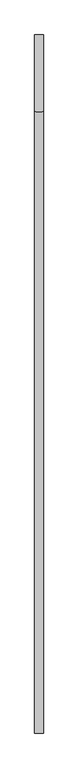
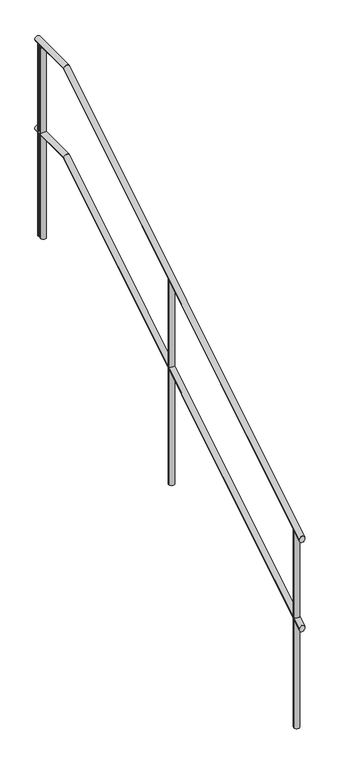
"""IFC4 building model written with IfcOpenShell, lengths in millimetres: railing geometry."""

import ifcopenshell
import ifcopenshell.guid

model = None  # the IFC model being written
_history = None  # IfcOwnerHistory: only IFC2X3 demands one
_inside = {}  # id of a spatial element -> (the spatial element, [elements in it])
_under = {}  # id of a project, library or spatial element -> (it, [spatial elements below it])
_declared = {}  # id of a project -> (the project, [libraries it declares])
_typed = {}  # id of a type object -> (the type object, [elements of that type])
_made_of = {}  # id of a material, layer set ... -> (it, [elements and type objects made of it])


def new_model(schema):
    """Start an empty IFC model of exactly this schema.

    Asked for "IFC4X3", IfcOpenShell would pick the latest addendum, in which some entities
    have other attributes; the version numbers below select the first issue.
    IFC2X3 requires an IfcOwnerHistory on every rooted entity: one is made here for all.
    """
    global model, _history
    if schema == "IFC4X3":
        model = ifcopenshell.file(schema_version=(4, 3, 0, 0))
    else:
        model = ifcopenshell.file(schema=schema)
    _inside.clear()
    _under.clear()
    _declared.clear()
    _typed.clear()
    _made_of.clear()
    _history = None
    if model.schema == "IFC2X3":
        org = make("IfcOrganization", Name="unknown")
        user = make(
            "IfcPersonAndOrganization",
            ThePerson=make("IfcPerson", FamilyName="unknown"),
            TheOrganization=org,
        )
        app = make(
            "IfcApplication",
            ApplicationDeveloper=org,
            Version="unknown",
            ApplicationFullName="unknown",
            ApplicationIdentifier="unknown",
        )
        _history = make(
            "IfcOwnerHistory",
            OwningUser=user,
            OwningApplication=app,
            ChangeAction="ADDED",
            CreationDate=0,
        )
    return model


def make(cls, **values):
    """One entity of the class cls with the attributes given. An attribute that is None is left unset."""
    return model.create_entity(
        cls, **{name: value for name, value in values.items() if value is not None}
    )


def rooted(cls, **values):
    """An entity with a GlobalId (a new one), such as an element, a storey or a relation."""
    return make(cls, GlobalId=ifcopenshell.guid.new(), OwnerHistory=_history, **values)


def si_unit(unit_type, name, prefix=None):
    """IfcSIUnit, for example si_unit("LENGTHUNIT", "METRE", prefix="MILLI")."""
    return make("IfcSIUnit", UnitType=unit_type, Prefix=prefix, Name=name)


def assignment(units):
    """IfcUnitAssignment: the units of a project."""
    return None if units is None else make("IfcUnitAssignment", Units=units)


def point(xyz):
    """IfcCartesianPoint."""
    return None if xyz is None else make("IfcCartesianPoint", Coordinates=xyz)


def direction(xyz):
    """IfcDirection."""
    return None if xyz is None else make("IfcDirection", DirectionRatios=xyz)


def frame(location, z_axis=None, x_axis=None):
    """IfcAxis2Placement3D, a coordinate frame: its origin and axes. An axis left out is left unset."""
    return make(
        "IfcAxis2Placement3D",
        Location=point(location),
        Axis=direction(z_axis),
        RefDirection=direction(x_axis),
    )


def frame_2d(location, x_axis=None):
    """IfcAxis2Placement2D, a coordinate frame in the plane: its origin and x axis."""
    return make(
        "IfcAxis2Placement2D", Location=point(location), RefDirection=direction(x_axis)
    )


def origin():
    """The frame at (0, 0, 0) with its axes left unset."""
    return frame((0.0, 0.0, 0.0))


def place(relative_to, where):
    """IfcLocalPlacement: puts the frame where relative to a parent placement (None: the world)."""
    return make(
        "IfcLocalPlacement", PlacementRelTo=relative_to, RelativePlacement=where
    )


def context(
    kind, dimensions, precision=None, world=None, true_north=None, identifier=None
):
    """IfcGeometricRepresentationContext, for example the 3D "Model" context."""
    return make(
        "IfcGeometricRepresentationContext",
        ContextIdentifier=identifier,
        ContextType=kind,
        CoordinateSpaceDimension=dimensions,
        Precision=precision,
        WorldCoordinateSystem=world,
        TrueNorth=true_north,
    )


def project(units=None, contexts=None):
    """IfcProject with its units and contexts."""
    return rooted(
        "IfcProject",
        Name="project",
        RepresentationContexts=contexts,
        UnitsInContext=assignment(units),
    )


def spatial(cls, under=None, at=None, **own):
    """A site, building, storey or space (cls), placed at a placement, below another one or the project."""
    s = rooted(cls, ObjectPlacement=at, **own)
    if under is not None:
        _under.setdefault(under.id(), (under, []))[1].append(s)
    return s


def circle_curve(where, radius):
    """IfcCircle in the frame where."""
    return make("IfcCircle", Position=where, Radius=radius)


def ellipse_curve(where, semi_axis1, semi_axis2):
    """IfcEllipse in the frame where."""
    return make(
        "IfcEllipse", Position=where, SemiAxis1=semi_axis1, SemiAxis2=semi_axis2
    )


def trimmed(basis, trim1, trim2, sense, master):
    """IfcTrimmedCurve: the piece of a basis curve between two trims."""
    return make(
        "IfcTrimmedCurve",
        BasisCurve=basis,
        Trim1=trim1,
        Trim2=trim2,
        SenseAgreement=sense,
        MasterRepresentation=master,
    )


def segment(curve, same_sense, transition):
    """IfcCompositeCurveSegment."""
    return make(
        "IfcCompositeCurveSegment",
        Transition=transition,
        SameSense=same_sense,
        ParentCurve=curve,
    )


def composite_curve(segments, self_intersect=None):
    """IfcCompositeCurve: segments joined end to end."""
    return make("IfcCompositeCurve", Segments=segments, SelfIntersect=self_intersect)


def outline(outer, holes=None, kind="AREA"):
    """IfcArbitraryClosedProfileDef: a profile drawn as a closed curve; with holes, ...WithVoids."""
    if holes is None:
        return make("IfcArbitraryClosedProfileDef", ProfileType=kind, OuterCurve=outer)
    return make(
        "IfcArbitraryProfileDefWithVoids",
        ProfileType=kind,
        OuterCurve=outer,
        InnerCurves=holes,
    )


def extrude(swept, where, along, depth):
    """IfcExtrudedAreaSolid: the profile swept, set in the frame where, extruded along a direction by depth."""
    return make(
        "IfcExtrudedAreaSolid",
        SweptArea=swept,
        Position=where,
        ExtrudedDirection=direction(along),
        Depth=depth,
    )


def shape(context_of_items, identifier, shape_type, items):
    """IfcShapeRepresentation: the items that make up one representation, for example the "Body"."""
    return make(
        "IfcShapeRepresentation",
        ContextOfItems=context_of_items,
        RepresentationIdentifier=identifier,
        RepresentationType=shape_type,
        Items=items,
    )


def source(mapping_origin, context_of_items, identifier, shape_type, items):
    """IfcRepresentationMap: a shape defined once, which mapped items show again and again."""
    return make(
        "IfcRepresentationMap",
        MappingOrigin=mapping_origin,
        MappedRepresentation=shape(context_of_items, identifier, shape_type, items),
    )


def transform(
    local_origin,
    x_axis=None,
    y_axis=None,
    z_axis=None,
    scale=None,
    scale2=None,
    scale3=None,
    uniform=True,
):
    """IfcCartesianTransformationOperator3D, or its non-uniform kind. x_axis, y_axis, z_axis: its Axis1, 2, 3."""
    if uniform:
        return make(
            "IfcCartesianTransformationOperator3D",
            Axis1=direction(x_axis),
            Axis2=direction(y_axis),
            LocalOrigin=point(local_origin),
            Scale=scale,
            Axis3=direction(z_axis),
        )
    return make(
        "IfcCartesianTransformationOperator3DnonUniform",
        Axis1=direction(x_axis),
        Axis2=direction(y_axis),
        LocalOrigin=point(local_origin),
        Scale=scale,
        Axis3=direction(z_axis),
        Scale2=scale2,
        Scale3=scale3,
    )


def mapped(mapping_source, mapping_target):
    """IfcMappedItem: shows the shape of a source again, moved by a transform."""
    return make(
        "IfcMappedItem", MappingSource=mapping_source, MappingTarget=mapping_target
    )


def made_of(thing, what):
    """Note that an element or type object is made of a material, layer set ...; save() writes the relation."""
    if what is not None:
        _made_of.setdefault(what.id(), (what, []))[1].append(thing)
    return thing


def element(
    cls,
    number,
    at=None,
    inside=None,
    cuts=None,
    type_object=None,
    material=None,
    context=None,
    identifier="Body",
    shape_type=None,
    held_by="IfcProductDefinitionShape",
    body=None,
    shapes=None,
    **own,
):
    """One element of the class cls, such as IfcWall. Its Tag is "e" and its number.

    at: its placement. inside: the storey or other place that contains it. cuts: it is an
    opening in that element (IfcRelVoidsElement). A single representation is given by context,
    identifier, shape_type and body (its items); several are given by shapes. held_by: the class
    of the entity that holds the representations. save() writes the other relations.
    """
    e = rooted(cls, Tag="e%d" % number, ObjectPlacement=at, **own)
    if body is not None:
        shapes = [shape(context, identifier, shape_type, body)]
    if shapes is not None:
        e.Representation = make(held_by, Representations=shapes)
    if inside is not None:
        _inside.setdefault(inside.id(), (inside, []))[1].append(e)
    if cuts is not None:
        rooted(
            "IfcRelVoidsElement", RelatingBuildingElement=cuts, RelatedOpeningElement=e
        )
    if type_object is not None:
        _typed.setdefault(type_object.id(), (type_object, []))[1].append(e)
    return made_of(e, material)


def aggregate(whole, parts):
    """IfcRelAggregates: a whole, such as a stair, and the parts it consists of."""
    return rooted("IfcRelAggregates", RelatingObject=whole, RelatedObjects=parts)


def save(model, path):
    """Write the relations noted so far, then the file.

    IfcRelAggregates (storeys below a building ...), IfcRelContainedInSpatialStructure (elements
    in a storey), IfcRelDefinesByType, IfcRelAssociatesMaterial and IfcRelDeclares: one each for
    every whole, place, type object, material and project.
    """
    for whole, parts in _under.values():
        aggregate(whole, parts)
    for where, things in _inside.values():
        rooted(
            "IfcRelContainedInSpatialStructure",
            RelatedElements=things,
            RelatingStructure=where,
        )
    for kind, things in _typed.values():
        rooted("IfcRelDefinesByType", RelatedObjects=things, RelatingType=kind)
    for what, things in _made_of.values():
        rooted("IfcRelAssociatesMaterial", RelatedObjects=things, RelatingMaterial=what)
    for by, libraries in _declared.values():
        rooted("IfcRelDeclares", RelatingContext=by, RelatedDefinitions=libraries)
    model.write(path)


def plane_surface(at):
    """IfcPlane: the flat surface through the origin of the frame at, square to its z axis."""
    return make("IfcPlane", Position=at)


def cylinder_surface(at, radius):
    """IfcCylindricalSurface: all points at the distance radius from the z axis of the frame at."""
    return make("IfcCylindricalSurface", Position=at, Radius=radius)


def advanced_brep(points, edges, surfaces, faces):
    """IfcAdvancedBrep: a solid bounded by faces that lie on surfaces and meet in shared edges.

    An edge is (start, end): straight between two places in points (the first is 0);
    or (start, end, curve); or (start, end, curve, False) where it runs against its curve.
    A face is (place in surfaces, loops), or (place, loops, False) where it looks against
    its surface's normal. A loop lists edges by number (the first is 1), with a minus sign
    where the edge is run from its end to its start. The first loop is the outer one.
    """
    corners = [point(p) for p in points]
    vertices = [make("IfcVertexPoint", VertexGeometry=c) for c in corners]
    made = []
    for start, end, *more in edges:
        made.append(
            make(
                "IfcEdgeCurve",
                EdgeStart=vertices[start],
                EdgeEnd=vertices[end],
                EdgeGeometry=more[0] if more else make("IfcPolyline", Points=[corners[start], corners[end]]),
                SameSense=more[1] if len(more) > 1 else True,
            )
        )
    hull = []
    for where, loops, *sense in faces:
        bounds = []
        for j, loop in enumerate(loops):
            ring = [make("IfcOrientedEdge", EdgeElement=made[abs(k) - 1], Orientation=k > 0) for k in loop]
            bounds.append(
                make(
                    "IfcFaceOuterBound" if j == 0 else "IfcFaceBound",
                    Bound=make("IfcEdgeLoop", EdgeList=ring),
                    Orientation=True,
                )
            )
        hull.append(make("IfcAdvancedFace", Bounds=bounds, FaceSurface=surfaces[where], SameSense=sense[0] if sense else True))
    return make("IfcAdvancedBrep", Outer=make("IfcClosedShell", CfsFaces=hull))


def railing_2704ba66(model_context):
    return source(origin(), model_context, "Body", "SolidModel", [
        advanced_brep(
        [(-1026.0, 45684.2482382, -450.9609787), (-1056.0, 45684.2482382, -450.9609787), (-1026.0, 47848.5050237, 885.0), (-1056.0, 47848.5050237, 885.0), (-1026.0, 48114.2482382, 885.0), (-1056.0, 48114.2482382, 885.0)],
        [
            (0, 1, ellipse_curve(frame((-1041.0, 45684.2482382, -450.9609787), z_axis=(0.0, -1.0, 0.0), x_axis=(0.0, 0.0, -1.0)), 17.6276454, 15.0)),
            (1, 0, ellipse_curve(frame((-1041.0, 45684.2482382, -450.9609787), z_axis=(0.0, -1.0, 0.0), x_axis=(0.0, 0.0, -1.0)), 17.6276454, 15.0)),
            (0, 2),
            (2, 3, ellipse_curve(frame((-1041.0, 47848.5050237, 885.0), z_axis=(0.0, -0.9620125025549409, -0.27300539358770887), x_axis=(0.0, 0.27300539358770864, -0.962012502554941)), 15.5923129, 15.0)),
            (3, 1),
            (3, 2, ellipse_curve(frame((-1041.0, 47848.5050237, 885.0), z_axis=(0.0, -0.9620125025549409, -0.27300539358770887), x_axis=(0.0, 0.27300539358770864, -0.962012502554941)), 15.5923129, 15.0)),
            (4, 5, circle_curve(frame((-1041.0, 48114.2482382, 885.0), z_axis=(0.0, 1.0, 0.0), x_axis=(-1.0, 0.0, 0.0)), 15.0)),
            (5, 4, circle_curve(frame((-1041.0, 48114.2482382, 885.0), z_axis=(0.0, 1.0, 0.0), x_axis=(-1.0, 0.0, 0.0)), 15.0)),
            (2, 4),
            (5, 3),
        ],
        [
            plane_surface(frame((-1041.0, 45684.2482382, -433.3333333), z_axis=(0.0, -1.0, 0.0), x_axis=(0.0, 0.0, 1.0))),
            cylinder_surface(frame((-1041.0, 45692.1272762, -446.097375), z_axis=(0.0, -0.8509361101440404, -0.5252692037926169), x_axis=(-1.0, 0.0, 0.0)), 15.0),
            plane_surface(frame((-1041.0, 48114.2482382, 900.0), z_axis=(0.0, 1.0, 0.0), x_axis=(0.0, 0.0, 1.0))),
            cylinder_surface(frame((-1041.0, 47844.2482382, 885.0), z_axis=(0.0, -1.0, 0.0), x_axis=(-1.0, 0.0, 0.0)), 15.0),
        ],
        [
            (0, [[1, 2]]),
            (1, [[-1, 3, 4, 5]]),
            (1, [[-2, -5, 6, -3]]),
            (2, [[7, 8]]),
            (3, [[-4, 9, -8, 10]]),
            (3, [[-6, -10, -7, -9]]),
        ],
    ),
        advanced_brep(
        [(-1026.0, 45684.2482382, 49.0390213), (-1056.0, 45684.2482382, 49.0390213), (-1026.0, 47848.5050237, 1385.0), (-1056.0, 47848.5050237, 1385.0), (-1026.0, 48114.2482382, 1385.0), (-1056.0, 48114.2482382, 1385.0)],
        [
            (0, 1, ellipse_curve(frame((-1041.0, 45684.2482382, 49.0390213), z_axis=(0.0, -1.0, 0.0), x_axis=(0.0, 0.0, -1.0)), 17.6276454, 15.0)),
            (1, 0, ellipse_curve(frame((-1041.0, 45684.2482382, 49.0390213), z_axis=(0.0, -1.0, 0.0), x_axis=(0.0, 0.0, -1.0)), 17.6276454, 15.0)),
            (0, 2),
            (2, 3, ellipse_curve(frame((-1041.0, 47848.5050237, 1385.0), z_axis=(0.0, -0.9620125025549409, -0.27300539358770887), x_axis=(0.0, 0.27300539358770864, -0.962012502554941)), 15.5923129, 15.0)),
            (3, 1),
            (3, 2, ellipse_curve(frame((-1041.0, 47848.5050237, 1385.0), z_axis=(0.0, -0.9620125025549409, -0.27300539358770887), x_axis=(0.0, 0.27300539358770864, -0.962012502554941)), 15.5923129, 15.0)),
            (4, 5, circle_curve(frame((-1041.0, 48114.2482382, 1385.0), z_axis=(0.0, 1.0, 0.0), x_axis=(-1.0, 0.0, 0.0)), 15.0)),
            (5, 4, circle_curve(frame((-1041.0, 48114.2482382, 1385.0), z_axis=(0.0, 1.0, 0.0), x_axis=(-1.0, 0.0, 0.0)), 15.0)),
            (2, 4),
            (5, 3),
        ],
        [
            plane_surface(frame((-1041.0, 45684.2482382, 66.6666667), z_axis=(0.0, -1.0, 0.0), x_axis=(0.0, 0.0, 1.0))),
            cylinder_surface(frame((-1041.0, 45692.1272762, 53.902625), z_axis=(0.0, -0.8509361101440404, -0.5252692037926169), x_axis=(-1.0, 0.0, 0.0)), 15.0),
            plane_surface(frame((-1041.0, 48114.2482382, 1400.0), z_axis=(0.0, 1.0, 0.0), x_axis=(0.0, 0.0, 1.0))),
            cylinder_surface(frame((-1041.0, 47844.2482382, 1385.0), z_axis=(0.0, -1.0, 0.0), x_axis=(-1.0, 0.0, 0.0)), 15.0),
        ],
        [
            (0, [[1, 2]]),
            (1, [[-1, 3, 4, 5]]),
            (1, [[-2, -5, 6, -3]]),
            (2, [[7, 8]]),
            (3, [[-4, 9, -8, 10]]),
            (3, [[-6, -10, -7, -9]]),
        ],
    ),
        extrude(outline(composite_curve([segment(trimmed(circle_curve(frame_2d((-1041.0, 48084.2482382)), 15.0), [point((-1026.0, 48084.2482382))], [point((-1056.0, 48084.2482382))], False, "CARTESIAN"), True, "CONTINUOUS"), segment(trimmed(circle_curve(frame_2d((-1041.0, 48084.2482382)), 15.0), [point((-1056.0, 48084.2482382))], [point((-1026.0, 48084.2482382))], False, "CARTESIAN"), True, "CONTINUOUS")], self_intersect=False)), frame((0.0, 0.0, 300.0), z_axis=(0.0, 0.0, 1.0), x_axis=(1.0, 0.0, 0.0)), (0.0, 0.0, 1.0), 1070.0),
        advanced_brep(
        [(-1056.0, 46884.2482382, 777.4074074), (-1026.0, 46884.2482382, 777.4074074), (-1026.0, 46884.2482382, -366.6666667), (-1056.0, 46884.2482382, -366.6666667)],
        [
            (0, 1, ellipse_curve(frame((-1041.0, 46884.2482382, 777.4074074), z_axis=(0.0, 0.5252692037926167, -0.8509361101440406), x_axis=(0.0, 0.8509361101440406, 0.5252692037926162)), 17.6276454, 15.0)),
            (1, 2),
            (2, 3, circle_curve(frame((-1041.0, 46884.2482382, -366.6666667), z_axis=(0.0, 0.0, 1.0), x_axis=(1.0, 0.0, 0.0)), 15.0)),
            (3, 0),
            (3, 2, circle_curve(frame((-1041.0, 46884.2482382, -366.6666667), z_axis=(0.0, 0.0, 1.0), x_axis=(1.0, 0.0, 0.0)), 15.0)),
            (1, 0, ellipse_curve(frame((-1041.0, 46884.2482382, 777.4074074), z_axis=(0.0, 0.5252692037926167, -0.8509361101440406), x_axis=(0.0, 0.8509361101440406, 0.5252692037926162)), 17.6276454, 15.0)),
        ],
        [
            cylinder_surface(frame((-1041.0, 46884.2482382, -466.6666667), z_axis=(0.0, 0.0, 1.0), x_axis=(1.0, 0.0, 0.0)), 15.0),
            plane_surface(frame((-1016.0, 46909.2482382, 792.8395062), z_axis=(0.0, -0.5252692037926167, 0.8509361101440406), x_axis=(-1.0, 0.0, 0.0))),
            plane_surface(frame((-1016.0, 46859.2482382, -366.6666667), z_axis=(0.0, 0.0, -1.0), x_axis=(-1.0, 0.0, 0.0))),
        ],
        [
            (0, [[1, 2, 3, 4]]),
            (0, [[5, -2, 6, -4]]),
            (1, [[-6, -1]]),
            (2, [[-5, -3]]),
        ],
    ),
        extrude(outline(composite_curve([segment(trimmed(circle_curve(frame_2d((-1041.0, 48064.2482382)), 15.0), [point((-1026.0, 48064.2482382))], [point((-1056.0, 48064.2482382))], False, "CARTESIAN"), True, "CONTINUOUS"), segment(trimmed(circle_curve(frame_2d((-1041.0, 48064.2482382)), 15.0), [point((-1056.0, 48064.2482382))], [point((-1026.0, 48064.2482382))], False, "CARTESIAN"), True, "CONTINUOUS")], self_intersect=False)), frame((0.0, 0.0, 300.0), z_axis=(0.0, 0.0, 1.0), x_axis=(1.0, 0.0, 0.0)), (0.0, 0.0, 1.0), 1070.0),
        advanced_brep(
        [(-1056.0, 45734.2482382, 67.5308642), (-1026.0, 45734.2482382, 67.5308642), (-1026.0, 45734.2482382, -1033.3333333), (-1056.0, 45734.2482382, -1033.3333333)],
        [
            (0, 1, ellipse_curve(frame((-1041.0, 45734.2482382, 67.5308642), z_axis=(0.0, 0.5252692037926167, -0.8509361101440406), x_axis=(0.0, 0.8509361101440406, 0.5252692037926162)), 17.6276454, 15.0)),
            (1, 2),
            (2, 3, circle_curve(frame((-1041.0, 45734.2482382, -1033.3333333), z_axis=(0.0, 0.0, 1.0), x_axis=(1.0, 0.0, 0.0)), 15.0)),
            (3, 0),
            (3, 2, circle_curve(frame((-1041.0, 45734.2482382, -1033.3333333), z_axis=(0.0, 0.0, 1.0), x_axis=(1.0, 0.0, 0.0)), 15.0)),
            (1, 0, ellipse_curve(frame((-1041.0, 45734.2482382, 67.5308642), z_axis=(0.0, 0.5252692037926167, -0.8509361101440406), x_axis=(0.0, 0.8509361101440406, 0.5252692037926162)), 17.6276454, 15.0)),
        ],
        [
            cylinder_surface(frame((-1041.0, 45734.2482382, -1133.3333333), z_axis=(0.0, 0.0, 1.0), x_axis=(1.0, 0.0, 0.0)), 15.0),
            plane_surface(frame((-1016.0, 45759.2482382, 82.962963), z_axis=(0.0, -0.5252692037926167, 0.8509361101440406), x_axis=(-1.0, 0.0, 0.0))),
            plane_surface(frame((-1016.0, 45709.2482382, -1033.3333333), z_axis=(0.0, 0.0, -1.0), x_axis=(-1.0, 0.0, 0.0))),
        ],
        [
            (0, [[1, 2, 3, 4]]),
            (0, [[5, -2, 6, -4]]),
            (1, [[-6, -1]]),
            (2, [[-5, -3]]),
        ],
    ),
    ])


if __name__ == "__main__":
    model = new_model("IFC4")
    model_context = context("Model", 3, world=origin())
    ifc_project = project(units=[si_unit("LENGTHUNIT", "METRE", prefix="MILLI")], contexts=[model_context])
    site = spatial("IfcSite", under=ifc_project)
    building = spatial("IfcBuilding", under=site)
    placement = place(None, origin())
    railing_shape = railing_2704ba66(model_context)
    element("IfcRailing", 1, at=placement, inside=building, context=model_context, shape_type="MappedRepresentation", body=[
        mapped(railing_shape, transform((0.0, 0.0, 0.0), x_axis=(1.0, 0.0, 0.0), y_axis=(0.0, 1.0, 0.0), z_axis=(0.0, 0.0, 1.0))),
    ])
    save(model, "model.ifc")
